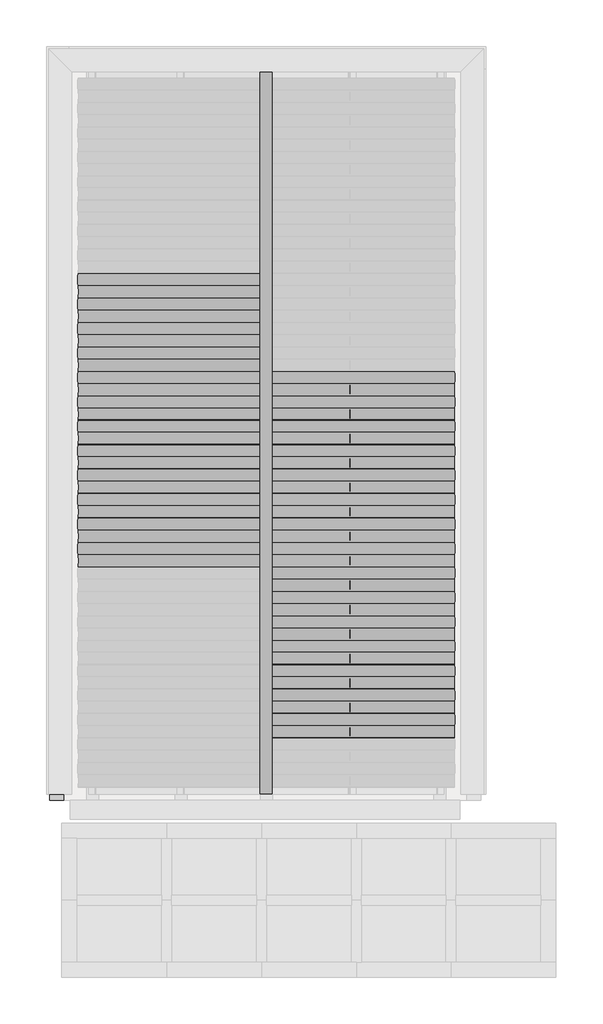
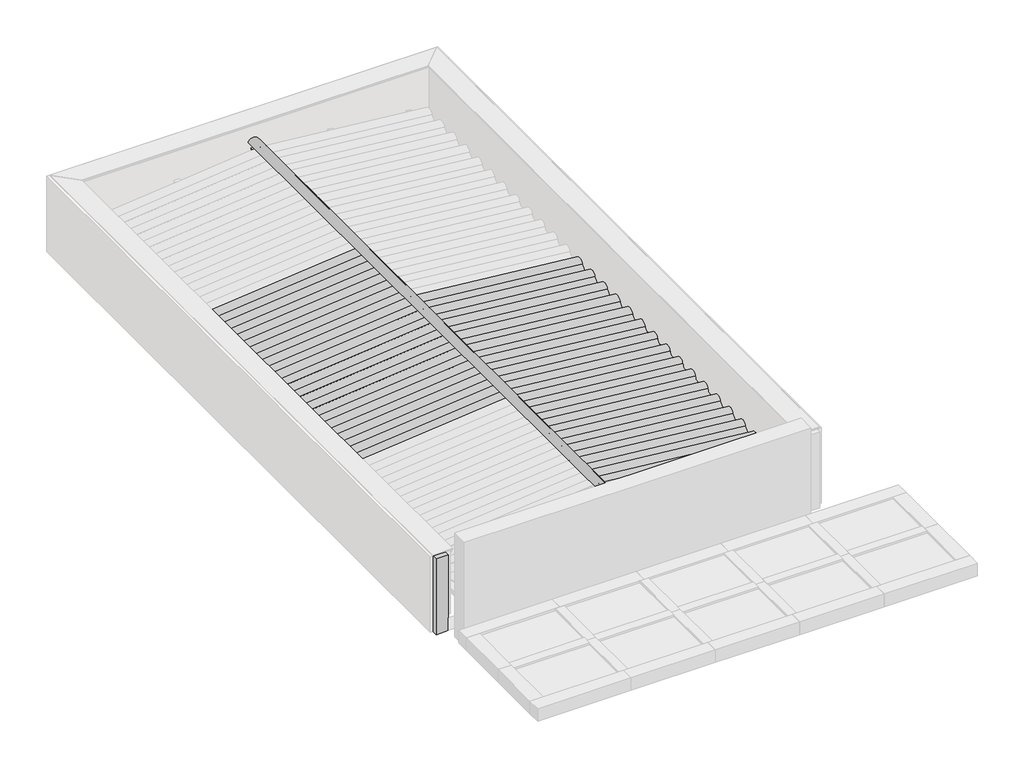
# One storey, part 2 of 3: 35 beams, 6 columns.
"""IFC4 building model written with IfcOpenShell, lengths in millimetres."""

import ifcopenshell
import ifcopenshell.guid

model = None  # the IFC model being written
_history = None  # IfcOwnerHistory: only IFC2X3 demands one
_inside = {}  # id of a spatial element -> (the spatial element, [elements in it])
_under = {}  # id of a project, library or spatial element -> (it, [spatial elements below it])
_declared = {}  # id of a project -> (the project, [libraries it declares])
_typed = {}  # id of a type object -> (the type object, [elements of that type])
_made_of = {}  # id of a material, layer set ... -> (it, [elements and type objects made of it])


def new_model(schema):
    """Start an empty IFC model of exactly this schema.

    Asked for "IFC4X3", IfcOpenShell would pick the latest addendum, in which some entities
    have other attributes; the version numbers below select the first issue.
    IFC2X3 requires an IfcOwnerHistory on every rooted entity: one is made here for all.
    """
    global model, _history
    if schema == "IFC4X3":
        model = ifcopenshell.file(schema_version=(4, 3, 0, 0))
    else:
        model = ifcopenshell.file(schema=schema)
    _inside.clear()
    _under.clear()
    _declared.clear()
    _typed.clear()
    _made_of.clear()
    _history = None
    if model.schema == "IFC2X3":
        org = make("IfcOrganization", Name="unknown")
        user = make(
            "IfcPersonAndOrganization",
            ThePerson=make("IfcPerson", FamilyName="unknown"),
            TheOrganization=org,
        )
        app = make(
            "IfcApplication",
            ApplicationDeveloper=org,
            Version="unknown",
            ApplicationFullName="unknown",
            ApplicationIdentifier="unknown",
        )
        _history = make(
            "IfcOwnerHistory",
            OwningUser=user,
            OwningApplication=app,
            ChangeAction="ADDED",
            CreationDate=0,
        )
    return model


def make(cls, **values):
    """One entity of the class cls with the attributes given. An attribute that is None is left unset."""
    return model.create_entity(
        cls, **{name: value for name, value in values.items() if value is not None}
    )


def rooted(cls, **values):
    """An entity with a GlobalId (a new one), such as an element, a storey or a relation."""
    return make(cls, GlobalId=ifcopenshell.guid.new(), OwnerHistory=_history, **values)


def si_unit(unit_type, name, prefix=None):
    """IfcSIUnit, for example si_unit("LENGTHUNIT", "METRE", prefix="MILLI")."""
    return make("IfcSIUnit", UnitType=unit_type, Prefix=prefix, Name=name)


def assignment(units):
    """IfcUnitAssignment: the units of a project."""
    return None if units is None else make("IfcUnitAssignment", Units=units)


def point(xyz):
    """IfcCartesianPoint."""
    return None if xyz is None else make("IfcCartesianPoint", Coordinates=xyz)


def direction(xyz):
    """IfcDirection."""
    return None if xyz is None else make("IfcDirection", DirectionRatios=xyz)


def frame(location, z_axis=None, x_axis=None):
    """IfcAxis2Placement3D, a coordinate frame: its origin and axes. An axis left out is left unset."""
    return make(
        "IfcAxis2Placement3D",
        Location=point(location),
        Axis=direction(z_axis),
        RefDirection=direction(x_axis),
    )


def frame_2d(location, x_axis=None):
    """IfcAxis2Placement2D, a coordinate frame in the plane: its origin and x axis."""
    return make(
        "IfcAxis2Placement2D", Location=point(location), RefDirection=direction(x_axis)
    )


def origin():
    """The frame at (0, 0, 0) with its axes left unset."""
    return frame((0.0, 0.0, 0.0))


def place(relative_to, where):
    """IfcLocalPlacement: puts the frame where relative to a parent placement (None: the world)."""
    return make(
        "IfcLocalPlacement", PlacementRelTo=relative_to, RelativePlacement=where
    )


def context(
    kind, dimensions, precision=None, world=None, true_north=None, identifier=None
):
    """IfcGeometricRepresentationContext, for example the 3D "Model" context."""
    return make(
        "IfcGeometricRepresentationContext",
        ContextIdentifier=identifier,
        ContextType=kind,
        CoordinateSpaceDimension=dimensions,
        Precision=precision,
        WorldCoordinateSystem=world,
        TrueNorth=true_north,
    )


def project(units=None, contexts=None):
    """IfcProject with its units and contexts."""
    return rooted(
        "IfcProject",
        Name="project",
        RepresentationContexts=contexts,
        UnitsInContext=assignment(units),
    )


def spatial(cls, under=None, at=None, **own):
    """A site, building, storey or space (cls), placed at a placement, below another one or the project."""
    s = rooted(cls, ObjectPlacement=at, **own)
    if under is not None:
        _under.setdefault(under.id(), (under, []))[1].append(s)
    return s


def polyline(points):
    """IfcPolyline through the points."""
    return make("IfcPolyline", Points=[point(p) for p in points])


def circle_curve(where, radius):
    """IfcCircle in the frame where."""
    return make("IfcCircle", Position=where, Radius=radius)


def trimmed(basis, trim1, trim2, sense, master):
    """IfcTrimmedCurve: the piece of a basis curve between two trims."""
    return make(
        "IfcTrimmedCurve",
        BasisCurve=basis,
        Trim1=trim1,
        Trim2=trim2,
        SenseAgreement=sense,
        MasterRepresentation=master,
    )


def segment(curve, same_sense, transition):
    """IfcCompositeCurveSegment."""
    return make(
        "IfcCompositeCurveSegment",
        Transition=transition,
        SameSense=same_sense,
        ParentCurve=curve,
    )


def composite_curve(segments, self_intersect=None):
    """IfcCompositeCurve: segments joined end to end."""
    return make("IfcCompositeCurve", Segments=segments, SelfIntersect=self_intersect)


def outline(outer, holes=None, kind="AREA"):
    """IfcArbitraryClosedProfileDef: a profile drawn as a closed curve; with holes, ...WithVoids."""
    if holes is None:
        return make("IfcArbitraryClosedProfileDef", ProfileType=kind, OuterCurve=outer)
    return make(
        "IfcArbitraryProfileDefWithVoids",
        ProfileType=kind,
        OuterCurve=outer,
        InnerCurves=holes,
    )


def extrude(swept, where, along, depth):
    """IfcExtrudedAreaSolid: the profile swept, set in the frame where, extruded along a direction by depth."""
    return make(
        "IfcExtrudedAreaSolid",
        SweptArea=swept,
        Position=where,
        ExtrudedDirection=direction(along),
        Depth=depth,
    )


def faces_of(points, faces, orient=None, outer=None):
    """IfcFace entities. A face is a list of loops; a loop is a list of indices into points, from 0.

    orient and outer hold one flag for each loop. By default every Orientation is true, the
    first loop of a face is its IfcFaceOuterBound and the others are IfcFaceBound.
    """
    made = []
    for i, loops in enumerate(faces):
        bounds = []
        for j, loop in enumerate(loops):
            is_outer = j == 0 if outer is None else outer[i][j]
            bounds.append(
                make(
                    "IfcFaceOuterBound" if is_outer else "IfcFaceBound",
                    Bound=make("IfcPolyLoop", Polygon=[points[k] for k in loop]),
                    Orientation=True if orient is None else orient[i][j],
                )
            )
        made.append(make("IfcFace", Bounds=bounds))
    return made


def faceted_brep(points, faces, orient=None, outer=None, voids=None):
    """IfcFacetedBrep: a solid bounded by flat faces; with voids (closed shells), ...WithVoids."""
    shared = [point(p) for p in points]
    hull = make("IfcClosedShell", CfsFaces=faces_of(shared, faces, orient, outer))
    if voids is None:
        return make("IfcFacetedBrep", Outer=hull)
    return make(
        "IfcFacetedBrepWithVoids",
        Outer=hull,
        Voids=[
            make(cls, CfsFaces=faces_of(shared, fs, o, b)) for cls, fs, o, b in voids
        ],
    )


def shape(context_of_items, identifier, shape_type, items):
    """IfcShapeRepresentation: the items that make up one representation, for example the "Body"."""
    return make(
        "IfcShapeRepresentation",
        ContextOfItems=context_of_items,
        RepresentationIdentifier=identifier,
        RepresentationType=shape_type,
        Items=items,
    )


def source(mapping_origin, context_of_items, identifier, shape_type, items):
    """IfcRepresentationMap: a shape defined once, which mapped items show again and again."""
    return make(
        "IfcRepresentationMap",
        MappingOrigin=mapping_origin,
        MappedRepresentation=shape(context_of_items, identifier, shape_type, items),
    )


def transform(
    local_origin,
    x_axis=None,
    y_axis=None,
    z_axis=None,
    scale=None,
    scale2=None,
    scale3=None,
    uniform=True,
):
    """IfcCartesianTransformationOperator3D, or its non-uniform kind. x_axis, y_axis, z_axis: its Axis1, 2, 3."""
    if uniform:
        return make(
            "IfcCartesianTransformationOperator3D",
            Axis1=direction(x_axis),
            Axis2=direction(y_axis),
            LocalOrigin=point(local_origin),
            Scale=scale,
            Axis3=direction(z_axis),
        )
    return make(
        "IfcCartesianTransformationOperator3DnonUniform",
        Axis1=direction(x_axis),
        Axis2=direction(y_axis),
        LocalOrigin=point(local_origin),
        Scale=scale,
        Axis3=direction(z_axis),
        Scale2=scale2,
        Scale3=scale3,
    )


def mapped(mapping_source, mapping_target):
    """IfcMappedItem: shows the shape of a source again, moved by a transform."""
    return make(
        "IfcMappedItem", MappingSource=mapping_source, MappingTarget=mapping_target
    )


def made_of(thing, what):
    """Note that an element or type object is made of a material, layer set ...; save() writes the relation."""
    if what is not None:
        _made_of.setdefault(what.id(), (what, []))[1].append(thing)
    return thing


def element(
    cls,
    number,
    at=None,
    inside=None,
    cuts=None,
    type_object=None,
    material=None,
    context=None,
    identifier="Body",
    shape_type=None,
    held_by="IfcProductDefinitionShape",
    body=None,
    shapes=None,
    **own,
):
    """One element of the class cls, such as IfcWall. Its Tag is "e" and its number.

    at: its placement. inside: the storey or other place that contains it. cuts: it is an
    opening in that element (IfcRelVoidsElement). A single representation is given by context,
    identifier, shape_type and body (its items); several are given by shapes. held_by: the class
    of the entity that holds the representations. save() writes the other relations.
    """
    e = rooted(cls, Tag="e%d" % number, ObjectPlacement=at, **own)
    if body is not None:
        shapes = [shape(context, identifier, shape_type, body)]
    if shapes is not None:
        e.Representation = make(held_by, Representations=shapes)
    if inside is not None:
        _inside.setdefault(inside.id(), (inside, []))[1].append(e)
    if cuts is not None:
        rooted(
            "IfcRelVoidsElement", RelatingBuildingElement=cuts, RelatedOpeningElement=e
        )
    if type_object is not None:
        _typed.setdefault(type_object.id(), (type_object, []))[1].append(e)
    return made_of(e, material)


def aggregate(whole, parts):
    """IfcRelAggregates: a whole, such as a stair, and the parts it consists of."""
    return rooted("IfcRelAggregates", RelatingObject=whole, RelatedObjects=parts)


def save(model, path):
    """Write the relations noted so far, then the file.

    IfcRelAggregates (storeys below a building ...), IfcRelContainedInSpatialStructure (elements
    in a storey), IfcRelDefinesByType, IfcRelAssociatesMaterial and IfcRelDeclares: one each for
    every whole, place, type object, material and project.
    """
    for whole, parts in _under.values():
        aggregate(whole, parts)
    for where, things in _inside.values():
        rooted(
            "IfcRelContainedInSpatialStructure",
            RelatedElements=things,
            RelatingStructure=where,
        )
    for kind, things in _typed.values():
        rooted("IfcRelDefinesByType", RelatedObjects=things, RelatingType=kind)
    for what, things in _made_of.values():
        rooted("IfcRelAssociatesMaterial", RelatedObjects=things, RelatingMaterial=what)
    for by, libraries in _declared.values():
        rooted("IfcRelDeclares", RelatingContext=by, RelatedDefinitions=libraries)
    model.write(path)


def cumeeira_telha_ondulada_fibrocimento_28917381(model_context):
    return source(origin(), model_context, "Body", "SweptSolid", [
        extrude(outline(composite_curve([segment(polyline([(58.3970135, 42.4437972), (53.9055884, 40.2467307)]), True, "CONTINUOUS"), segment(trimmed(circle_curve(frame_2d((-1.6029865, 13.0936483)), 61.7939461), [point((53.9055884, 40.2467307))], [point((-57.1115615, 40.2467307))], True, "CARTESIAN"), True, "CONTINUOUS"), segment(polyline([(-57.1115615, 40.2467307), (-61.6029865, 42.4437972)]), True, "CONTINUOUS"), segment(trimmed(circle_curve(frame_2d((-1.6029865, 13.0936483)), 66.7939461), [point((-61.6029865, 42.4437972))], [point((58.3970135, 42.4437972))], False, "CARTESIAN"), True, "CONTINUOUS")], self_intersect=False)), frame((-3626.5, 0.0, 0.0), z_axis=(1.0, 0.0, 0.0), x_axis=(0.0, 1.0, 0.0)), (0.0, 0.0, 1.0), 7253.0),
    ])


def viga_cumeeira_6x16cm_d80f05ee(model_context):
    return source(origin(), model_context, "Body", "SweptSolid", [
        extrude(outline(polyline([(3626.5, 30.0), (3626.5, -30.0), (-3626.5, -30.0), (-3626.5, 30.0), (3626.5, 30.0)])), frame((0.0, 0.0, -80.0), z_axis=(0.0, 0.0, 1.0), x_axis=(1.0, 0.0, 0.0)), (0.0, 0.0, 1.0), 160.0),
    ])


def column_1cffec27(model_context):
    return source(origin(), model_context, "Body", "SweptSolid", [
        extrude(outline(polyline([(30.0, 80.0), (30.0, -80.0), (-30.0, -80.0), (-30.0, 80.0), (30.0, 80.0)])), frame((0.0, 0.0, 3110.0), z_axis=(0.0, 0.0, 1.0), x_axis=(1.0, 0.0, 0.0)), (0.0, 0.0, 1.0), 238.0),
    ])


def column_35730ad5(model_context):
    return source(origin(), model_context, "Body", "SweptSolid", [
        extrude(outline(polyline([(30.0, 80.0), (30.0, -80.0), (-30.0, -80.0), (-30.0, 80.0), (30.0, 80.0)])), frame((0.0, 0.0, 3110.0), z_axis=(0.0, 0.0, 1.0), x_axis=(1.0, 0.0, 0.0)), (0.0, 0.0, 1.0), 197.9),
    ])


def column_00c463e4(model_context):
    return source(origin(), model_context, "Body", "SweptSolid", [
        extrude(outline(polyline([(30.0, 80.0), (30.0, -80.0), (-30.0, -80.0), (-30.0, 80.0), (30.0, 80.0)])), frame((0.0, 0.0, 3110.0), z_axis=(0.0, 0.0, 1.0), x_axis=(1.0, 0.0, 0.0)), (0.0, 0.0, 1.0), 109.8),
    ])


model = new_model("IFC4")

# Units and contexts
model_context = context("Model", 3, world=origin())
ifc_project = project(units=[si_unit("LENGTHUNIT", "METRE", prefix="MILLI")], contexts=[model_context])

# Site, building, storey
site = spatial("IfcSite", under=ifc_project)
building = spatial("IfcBuilding", under=site)
storey = spatial("IfcBuildingStorey", under=building, Name="COB. GARAGEM", Elevation=3050.0)

# Beams
placement = place(None, origin())
element("IfcBeam", 1, ObjectType="Madeira de lei : Berço 6x12cm", at=placement, inside=storey, context=model_context, shape_type="SweptSolid", body=[
    extrude(outline(polyline([(-9620.281307, 4423.9300153), (-9500.281307, 4423.9300153), (-9500.281307, 2423.9300153), (-9620.281307, 2423.9300153), (-9620.281307, 4423.9300153)])), frame((0.0, 0.0, 3050.0), z_axis=(0.0, 0.0, 1.0), x_axis=(1.0, 0.0, 0.0)), (0.0, 0.0, 1.0), 60.0),
])
element("IfcBeam", 2, ObjectType="Madeira de lei : Berço 6x12cm", at=placement, inside=storey, context=model_context, shape_type="SweptSolid", body=[
    extrude(outline(polyline([(-9620.281307, 2423.9300153), (-9500.281307, 2423.9300153), (-9500.281307, 423.9300153), (-9620.281307, 423.9300153), (-9620.281307, 2423.9300153)])), frame((0.0, 0.0, 3050.0), z_axis=(0.0, 0.0, 1.0), x_axis=(1.0, 0.0, 0.0)), (0.0, 0.0, 1.0), 60.0),
])
element("IfcBeam", 3, ObjectType="Madeira de lei : Berço 6x12cm", at=placement, inside=storey, context=model_context, shape_type="SweptSolid", body=[
    extrude(outline(polyline([(-8767.0824227, 4423.9300153), (-8647.0824227, 4423.9300153), (-8647.0824227, 2423.9300153), (-8767.0824227, 2423.9300153), (-8767.0824227, 4423.9300153)])), frame((0.0, 0.0, 3050.0), z_axis=(0.0, 0.0, 1.0), x_axis=(1.0, 0.0, 0.0)), (0.0, 0.0, 1.0), 60.0),
])
element("IfcBeam", 4, ObjectType="Madeira de lei : Berço 6x12cm", at=placement, inside=storey, context=model_context, shape_type="SweptSolid", body=[
    extrude(outline(polyline([(-10473.4801913, 4423.9300153), (-10353.4801913, 4423.9300153), (-10353.4801913, 2423.9300153), (-10473.4801913, 2423.9300153), (-10473.4801913, 4423.9300153)])), frame((0.0, 0.0, 3050.0), z_axis=(0.0, 0.0, 1.0), x_axis=(1.0, 0.0, 0.0)), (0.0, 0.0, 1.0), 60.0),
])
element("IfcBeam", 5, ObjectType="Madeira de lei : Berço 6x12cm", at=placement, inside=storey, context=model_context, shape_type="SweptSolid", body=[
    extrude(outline(polyline([(-11356.5301913, 4423.9300153), (-11236.5301913, 4423.9300153), (-11236.5301913, 2423.9300153), (-11356.5301913, 2423.9300153), (-11356.5301913, 4423.9300153)])), frame((0.0, 0.0, 3050.0), z_axis=(0.0, 0.0, 1.0), x_axis=(1.0, 0.0, 0.0)), (0.0, 0.0, 1.0), 60.0),
])
cumeeira_telha_ondulada_fibrocimento_shape = cumeeira_telha_ondulada_fibrocimento_28917381(model_context)
element("IfcBeam", 6, ObjectType="Cumeeira Telha Ondulada : Fibrocimento", at=placement, inside=storey, context=model_context, shape_type="MappedRepresentation", body=[
    mapped(cumeeira_telha_ondulada_fibrocimento_shape, transform((-9560.281307, 3455.9300153, 3545.9751229), x_axis=(0.0, -1.0, 0.0), y_axis=(1.0, 0.0, 0.0), z_axis=(0.0, 0.0, 1.0))),
])
element("IfcBeam", 7, ObjectType="TQS - Viga retangular : 14.0 x 90.0", at=placement, inside=storey, context=model_context, shape_type="Brep", body=[
    faceted_brep([(-11590.281307, 7084.4300153, 3800.0), (-11730.281307, 7084.4300153, 3800.0), (-11730.281307, -234.5699847, 3800.0), (-11590.281307, -234.5699847, 3800.0), (-11590.281307, 7084.4300153, 2900.0), (-11590.281307, 7084.4300153, 3050.0), (-11590.281307, -234.5699847, 3050.0), (-11590.281307, -234.5699847, 2900.0), (-11730.281307, 7084.4300153, 2900.0), (-11730.281307, -234.5699847, 2900.0)], [[[0, 1, 2, 3]], [[4, 5, 0, 3, 6, 7]], [[8, 4, 7, 9]], [[1, 8, 9, 2]], [[2, 9, 7, 6, 3]], [[1, 0, 5, 4, 8]]]),
])
element("IfcBeam", 8, ObjectType="Telha Ondulada : Fibrocimento", at=placement, inside=storey, context=model_context, shape_type="SweptSolid", body=[
    extrude(outline(composite_curve([segment(trimmed(circle_curve(frame_2d((-58.7002979, -53.2060538)), 66.7939461), [point((-29.350149, 6.7939462))], [point((-29.350149, -113.2060538))], False, "CARTESIAN"), True, "CONTINUOUS"), segment(polyline([(-29.350149, -113.2060538), (-31.5472155, -108.7146288)]), True, "CONTINUOUS"), segment(trimmed(circle_curve(frame_2d((-58.7002979, -53.2060538)), 61.7939461), [point((-31.5472155, -108.7146288))], [point((-31.5472155, 2.3025211))], True, "CARTESIAN"), True, "CONTINUOUS"), segment(trimmed(circle_curve(frame_2d((0.0, 66.7939462)), 71.7939461), [point((-31.5472155, 2.3025211))], [point((-31.5472155, 131.2853712))], False, "CARTESIAN"), True, "CONTINUOUS"), segment(polyline([(-31.5472155, 131.2853712), (-29.350149, 126.7939462)]), True, "CONTINUOUS"), segment(trimmed(circle_curve(frame_2d((0.0, 66.7939462)), 66.7939461), [point((-29.350149, 126.7939462))], [point((-29.350149, 6.7939462))], True, "CARTESIAN"), True, "CONTINUOUS")], self_intersect=False)), frame((-11446.918865, 2229.326948, 3394.3067746), z_axis=(0.9950371902099892, 0.0, 0.09950371902099919), x_axis=(-0.09950371902099919, 0.0, 0.9950371902099892)), (0.0, 0.0, 1.0), 1886.8678854),
])
element("IfcBeam", 9, ObjectType="Telha Ondulada : Fibrocimento", at=placement, inside=storey, context=model_context, shape_type="SweptSolid", body=[
    extrude(outline(composite_curve([segment(trimmed(circle_curve(frame_2d((-58.7002979, -53.2060538)), 66.7939461), [point((-29.350149, 6.7939462))], [point((-29.350149, -113.2060538))], False, "CARTESIAN"), True, "CONTINUOUS"), segment(polyline([(-29.350149, -113.2060538), (-31.5472155, -108.7146288)]), True, "CONTINUOUS"), segment(trimmed(circle_curve(frame_2d((-58.7002979, -53.2060538)), 61.7939461), [point((-31.5472155, -108.7146288))], [point((-31.5472155, 2.3025211))], True, "CARTESIAN"), True, "CONTINUOUS"), segment(trimmed(circle_curve(frame_2d((0.0, 66.7939462)), 71.7939461), [point((-31.5472155, 2.3025211))], [point((-31.5472155, 131.2853712))], False, "CARTESIAN"), True, "CONTINUOUS"), segment(polyline([(-31.5472155, 131.2853712), (-29.350149, 126.7939462)]), True, "CONTINUOUS"), segment(trimmed(circle_curve(frame_2d((0.0, 66.7939462)), 66.7939461), [point((-29.350149, 126.7939462))], [point((-29.350149, 6.7939462))], True, "CARTESIAN"), True, "CONTINUOUS")], self_intersect=False)), frame((-11446.918865, 2473.826948, 3394.3067746), z_axis=(0.9950371902099892, 0.0, 0.09950371902099932), x_axis=(-0.09950371902099932, 0.0, 0.9950371902099892)), (0.0, 0.0, 1.0), 1886.8678854),
])
element("IfcBeam", 10, ObjectType="Telha Ondulada : Fibrocimento", at=placement, inside=storey, context=model_context, shape_type="SweptSolid", body=[
    extrude(outline(composite_curve([segment(trimmed(circle_curve(frame_2d((-58.7002979, -53.2060538)), 66.7939461), [point((-29.350149, 6.7939462))], [point((-29.350149, -113.2060538))], False, "CARTESIAN"), True, "CONTINUOUS"), segment(polyline([(-29.350149, -113.2060538), (-31.5472155, -108.7146288)]), True, "CONTINUOUS"), segment(trimmed(circle_curve(frame_2d((-58.7002979, -53.2060538)), 61.7939461), [point((-31.5472155, -108.7146288))], [point((-31.5472155, 2.3025211))], True, "CARTESIAN"), True, "CONTINUOUS"), segment(trimmed(circle_curve(frame_2d((0.0, 66.7939462)), 71.7939461), [point((-31.5472155, 2.3025211))], [point((-31.5472155, 131.2853712))], False, "CARTESIAN"), True, "CONTINUOUS"), segment(polyline([(-31.5472155, 131.2853712), (-29.350149, 126.7939462)]), True, "CONTINUOUS"), segment(trimmed(circle_curve(frame_2d((0.0, 66.7939462)), 66.7939461), [point((-29.350149, 126.7939462))], [point((-29.350149, 6.7939462))], True, "CARTESIAN"), True, "CONTINUOUS")], self_intersect=False)), frame((-11446.918865, 2718.326948, 3394.3067746), z_axis=(0.9950371902099892, 0.0, 0.09950371902099937), x_axis=(-0.09950371902099937, 0.0, 0.9950371902099892)), (0.0, 0.0, 1.0), 1886.8678854),
])
element("IfcBeam", 11, ObjectType="Telha Ondulada : Fibrocimento", at=placement, inside=storey, context=model_context, shape_type="SweptSolid", body=[
    extrude(outline(composite_curve([segment(trimmed(circle_curve(frame_2d((-58.7002979, -53.2060538)), 66.7939461), [point((-29.350149, 6.7939462))], [point((-29.350149, -113.2060538))], False, "CARTESIAN"), True, "CONTINUOUS"), segment(polyline([(-29.350149, -113.2060538), (-31.5472155, -108.7146288)]), True, "CONTINUOUS"), segment(trimmed(circle_curve(frame_2d((-58.7002979, -53.2060538)), 61.7939461), [point((-31.5472155, -108.7146288))], [point((-31.5472155, 2.3025211))], True, "CARTESIAN"), True, "CONTINUOUS"), segment(trimmed(circle_curve(frame_2d((0.0, 66.7939462)), 71.7939461), [point((-31.5472155, 2.3025211))], [point((-31.5472155, 131.2853712))], False, "CARTESIAN"), True, "CONTINUOUS"), segment(polyline([(-31.5472155, 131.2853712), (-29.350149, 126.7939462)]), True, "CONTINUOUS"), segment(trimmed(circle_curve(frame_2d((0.0, 66.7939462)), 66.7939461), [point((-29.350149, 126.7939462))], [point((-29.350149, 6.7939462))], True, "CARTESIAN"), True, "CONTINUOUS")], self_intersect=False)), frame((-11446.918865, 2962.826948, 3394.3067746), z_axis=(0.9950371902099892, 0.0, 0.09950371902099943), x_axis=(-0.09950371902099943, 0.0, 0.9950371902099892)), (0.0, 0.0, 1.0), 1886.8678854),
])
element("IfcBeam", 12, ObjectType="Telha Ondulada : Fibrocimento", at=placement, inside=storey, context=model_context, shape_type="SweptSolid", body=[
    extrude(outline(composite_curve([segment(trimmed(circle_curve(frame_2d((-58.7002979, -53.2060538)), 66.7939461), [point((-29.350149, 6.7939462))], [point((-29.350149, -113.2060538))], False, "CARTESIAN"), True, "CONTINUOUS"), segment(polyline([(-29.350149, -113.2060538), (-31.5472155, -108.7146288)]), True, "CONTINUOUS"), segment(trimmed(circle_curve(frame_2d((-58.7002979, -53.2060538)), 61.7939461), [point((-31.5472155, -108.7146288))], [point((-31.5472155, 2.3025211))], True, "CARTESIAN"), True, "CONTINUOUS"), segment(trimmed(circle_curve(frame_2d((0.0, 66.7939462)), 71.7939461), [point((-31.5472155, 2.3025211))], [point((-31.5472155, 131.2853712))], False, "CARTESIAN"), True, "CONTINUOUS"), segment(polyline([(-31.5472155, 131.2853712), (-29.350149, 126.7939462)]), True, "CONTINUOUS"), segment(trimmed(circle_curve(frame_2d((0.0, 66.7939462)), 66.7939461), [point((-29.350149, 126.7939462))], [point((-29.350149, 6.7939462))], True, "CARTESIAN"), True, "CONTINUOUS")], self_intersect=False)), frame((-11446.918865, 3207.326948, 3394.3067746), z_axis=(0.9950371902099892, 0.0, 0.09950371902099954), x_axis=(-0.09950371902099954, 0.0, 0.9950371902099892)), (0.0, 0.0, 1.0), 1886.8678854),
])
element("IfcBeam", 13, ObjectType="Telha Ondulada : Fibrocimento", at=placement, inside=storey, context=model_context, shape_type="SweptSolid", body=[
    extrude(outline(composite_curve([segment(trimmed(circle_curve(frame_2d((-58.7002979, -53.2060538)), 66.7939461), [point((-29.350149, 6.7939462))], [point((-29.350149, -113.2060538))], False, "CARTESIAN"), True, "CONTINUOUS"), segment(polyline([(-29.350149, -113.2060538), (-31.5472155, -108.7146288)]), True, "CONTINUOUS"), segment(trimmed(circle_curve(frame_2d((-58.7002979, -53.2060538)), 61.7939461), [point((-31.5472155, -108.7146288))], [point((-31.5472155, 2.3025211))], True, "CARTESIAN"), True, "CONTINUOUS"), segment(trimmed(circle_curve(frame_2d((0.0, 66.7939462)), 71.7939461), [point((-31.5472155, 2.3025211))], [point((-31.5472155, 131.2853712))], False, "CARTESIAN"), True, "CONTINUOUS"), segment(polyline([(-31.5472155, 131.2853712), (-29.350149, 126.7939462)]), True, "CONTINUOUS"), segment(trimmed(circle_curve(frame_2d((0.0, 66.7939462)), 66.7939461), [point((-29.350149, 126.7939462))], [point((-29.350149, 6.7939462))], True, "CARTESIAN"), True, "CONTINUOUS")], self_intersect=False)), frame((-11446.918865, 3451.826948, 3394.3067746), z_axis=(0.9950371902099892, 0.0, 0.09950371902099937), x_axis=(-0.09950371902099937, 0.0, 0.9950371902099892)), (0.0, 0.0, 1.0), 1886.8678854),
])
element("IfcBeam", 14, ObjectType="Telha Ondulada : Fibrocimento", at=placement, inside=storey, context=model_context, shape_type="SweptSolid", body=[
    extrude(outline(composite_curve([segment(trimmed(circle_curve(frame_2d((-58.7002979, -53.2060538)), 66.7939461), [point((-29.350149, 6.7939462))], [point((-29.350149, -113.2060538))], False, "CARTESIAN"), True, "CONTINUOUS"), segment(polyline([(-29.350149, -113.2060538), (-31.5472155, -108.7146288)]), True, "CONTINUOUS"), segment(trimmed(circle_curve(frame_2d((-58.7002979, -53.2060538)), 61.7939461), [point((-31.5472155, -108.7146288))], [point((-31.5472155, 2.3025211))], True, "CARTESIAN"), True, "CONTINUOUS"), segment(trimmed(circle_curve(frame_2d((0.0, 66.7939462)), 71.7939461), [point((-31.5472155, 2.3025211))], [point((-31.5472155, 131.2853712))], False, "CARTESIAN"), True, "CONTINUOUS"), segment(polyline([(-31.5472155, 131.2853712), (-29.350149, 126.7939462)]), True, "CONTINUOUS"), segment(trimmed(circle_curve(frame_2d((0.0, 66.7939462)), 66.7939461), [point((-29.350149, 126.7939462))], [point((-29.350149, 6.7939462))], True, "CARTESIAN"), True, "CONTINUOUS")], self_intersect=False)), frame((-11446.918865, 3696.326948, 3394.3067746), z_axis=(0.9950371902099892, 0.0, 0.09950371902099914), x_axis=(-0.09950371902099914, 0.0, 0.9950371902099892)), (0.0, 0.0, 1.0), 1886.8678854),
])
element("IfcBeam", 15, ObjectType="Telha Ondulada : Fibrocimento", at=placement, inside=storey, context=model_context, shape_type="SweptSolid", body=[
    extrude(outline(composite_curve([segment(trimmed(circle_curve(frame_2d((-58.7002979, -53.2060538)), 66.7939461), [point((-29.350149, 6.7939462))], [point((-29.350149, -113.2060538))], False, "CARTESIAN"), True, "CONTINUOUS"), segment(polyline([(-29.350149, -113.2060538), (-31.5472155, -108.7146288)]), True, "CONTINUOUS"), segment(trimmed(circle_curve(frame_2d((-58.7002979, -53.2060538)), 61.7939461), [point((-31.5472155, -108.7146288))], [point((-31.5472155, 2.3025211))], True, "CARTESIAN"), True, "CONTINUOUS"), segment(trimmed(circle_curve(frame_2d((0.0, 66.7939462)), 71.7939461), [point((-31.5472155, 2.3025211))], [point((-31.5472155, 131.2853712))], False, "CARTESIAN"), True, "CONTINUOUS"), segment(polyline([(-31.5472155, 131.2853712), (-29.350149, 126.7939462)]), True, "CONTINUOUS"), segment(trimmed(circle_curve(frame_2d((0.0, 66.7939462)), 66.7939461), [point((-29.350149, 126.7939462))], [point((-29.350149, 6.7939462))], True, "CARTESIAN"), True, "CONTINUOUS")], self_intersect=False)), frame((-11446.918865, 3940.826948, 3394.3067746), z_axis=(0.9950371902099892, 0.0, 0.09950371902099948), x_axis=(-0.09950371902099948, 0.0, 0.9950371902099892)), (0.0, 0.0, 1.0), 1886.8678854),
])
element("IfcBeam", 16, ObjectType="Telha Ondulada : Fibrocimento", at=placement, inside=storey, context=model_context, shape_type="SweptSolid", body=[
    extrude(outline(composite_curve([segment(trimmed(circle_curve(frame_2d((-58.7002979, -53.2060538)), 66.7939461), [point((-29.350149, 6.7939462))], [point((-29.350149, -113.2060538))], False, "CARTESIAN"), True, "CONTINUOUS"), segment(polyline([(-29.350149, -113.2060538), (-31.5472155, -108.7146288)]), True, "CONTINUOUS"), segment(trimmed(circle_curve(frame_2d((-58.7002979, -53.2060538)), 61.7939461), [point((-31.5472155, -108.7146288))], [point((-31.5472155, 2.3025211))], True, "CARTESIAN"), True, "CONTINUOUS"), segment(trimmed(circle_curve(frame_2d((0.0, 66.7939462)), 71.7939461), [point((-31.5472155, 2.3025211))], [point((-31.5472155, 131.2853712))], False, "CARTESIAN"), True, "CONTINUOUS"), segment(polyline([(-31.5472155, 131.2853712), (-29.350149, 126.7939462)]), True, "CONTINUOUS"), segment(trimmed(circle_curve(frame_2d((0.0, 66.7939462)), 66.7939461), [point((-29.350149, 126.7939462))], [point((-29.350149, 6.7939462))], True, "CARTESIAN"), True, "CONTINUOUS")], self_intersect=False)), frame((-11446.918865, 4185.326948, 3394.3067746), z_axis=(0.9950371902099892, 0.0, 0.09950371902099932), x_axis=(-0.09950371902099932, 0.0, 0.9950371902099892)), (0.0, 0.0, 1.0), 1886.8678854),
])
element("IfcBeam", 17, ObjectType="Telha Ondulada : Fibrocimento", at=placement, inside=storey, context=model_context, shape_type="SweptSolid", body=[
    extrude(outline(composite_curve([segment(trimmed(circle_curve(frame_2d((-58.7002979, -53.2060538)), 66.7939461), [point((-29.350149, 6.7939462))], [point((-29.350149, -113.2060538))], False, "CARTESIAN"), True, "CONTINUOUS"), segment(polyline([(-29.350149, -113.2060538), (-31.5472155, -108.7146288)]), True, "CONTINUOUS"), segment(trimmed(circle_curve(frame_2d((-58.7002979, -53.2060538)), 61.7939461), [point((-31.5472155, -108.7146288))], [point((-31.5472155, 2.3025211))], True, "CARTESIAN"), True, "CONTINUOUS"), segment(trimmed(circle_curve(frame_2d((0.0, 66.7939462)), 71.7939461), [point((-31.5472155, 2.3025211))], [point((-31.5472155, 131.2853712))], False, "CARTESIAN"), True, "CONTINUOUS"), segment(polyline([(-31.5472155, 131.2853712), (-29.350149, 126.7939462)]), True, "CONTINUOUS"), segment(trimmed(circle_curve(frame_2d((0.0, 66.7939462)), 66.7939461), [point((-29.350149, 126.7939462))], [point((-29.350149, 6.7939462))], True, "CARTESIAN"), True, "CONTINUOUS")], self_intersect=False)), frame((-11446.918865, 4429.826948, 3394.3067746), z_axis=(0.9950371902099892, 0.0, 0.09950371902099943), x_axis=(-0.09950371902099943, 0.0, 0.9950371902099892)), (0.0, 0.0, 1.0), 1886.8678854),
])
element("IfcBeam", 18, ObjectType="Telha Ondulada : Fibrocimento", at=placement, inside=storey, context=model_context, shape_type="SweptSolid", body=[
    extrude(outline(composite_curve([segment(trimmed(circle_curve(frame_2d((-58.7002979, -53.2060538)), 66.7939461), [point((-29.350149, 6.7939462))], [point((-29.350149, -113.2060538))], False, "CARTESIAN"), True, "CONTINUOUS"), segment(polyline([(-29.350149, -113.2060538), (-31.5472155, -108.7146288)]), True, "CONTINUOUS"), segment(trimmed(circle_curve(frame_2d((-58.7002979, -53.2060538)), 61.7939461), [point((-31.5472155, -108.7146288))], [point((-31.5472155, 2.3025211))], True, "CARTESIAN"), True, "CONTINUOUS"), segment(trimmed(circle_curve(frame_2d((0.0, 66.7939462)), 71.7939461), [point((-31.5472155, 2.3025211))], [point((-31.5472155, 131.2853712))], False, "CARTESIAN"), True, "CONTINUOUS"), segment(polyline([(-31.5472155, 131.2853712), (-29.350149, 126.7939462)]), True, "CONTINUOUS"), segment(trimmed(circle_curve(frame_2d((0.0, 66.7939462)), 66.7939461), [point((-29.350149, 126.7939462))], [point((-29.350149, 6.7939462))], True, "CARTESIAN"), True, "CONTINUOUS")], self_intersect=False)), frame((-11446.918865, 4674.326948, 3394.3067746), z_axis=(0.9950371902099892, 0.0, 0.09950371902099943), x_axis=(-0.09950371902099943, 0.0, 0.9950371902099892)), (0.0, 0.0, 1.0), 1886.8678854),
])
element("IfcBeam", 19, ObjectType="Telha Ondulada : Fibrocimento", at=placement, inside=storey, context=model_context, shape_type="SweptSolid", body=[
    extrude(outline(composite_curve([segment(trimmed(circle_curve(frame_2d((-58.7002979, -53.2060538)), 66.7939461), [point((-29.350149, 6.7939462))], [point((-29.350149, -113.2060538))], False, "CARTESIAN"), True, "CONTINUOUS"), segment(polyline([(-29.350149, -113.2060538), (-31.5472155, -108.7146288)]), True, "CONTINUOUS"), segment(trimmed(circle_curve(frame_2d((-58.7002979, -53.2060538)), 61.7939461), [point((-31.5472155, -108.7146288))], [point((-31.5472155, 2.3025211))], True, "CARTESIAN"), True, "CONTINUOUS"), segment(trimmed(circle_curve(frame_2d((0.0, 66.7939462)), 71.7939461), [point((-31.5472155, 2.3025211))], [point((-31.5472155, 131.2853712))], False, "CARTESIAN"), True, "CONTINUOUS"), segment(polyline([(-31.5472155, 131.2853712), (-29.350149, 126.7939462)]), True, "CONTINUOUS"), segment(trimmed(circle_curve(frame_2d((0.0, 66.7939462)), 66.7939461), [point((-29.350149, 126.7939462))], [point((-29.350149, 6.7939462))], True, "CARTESIAN"), True, "CONTINUOUS")], self_intersect=False)), frame((-11446.918865, 4918.826948, 3394.3067746), z_axis=(0.9950371902099892, 0.0, 0.09950371902099903), x_axis=(-0.09950371902099903, 0.0, 0.9950371902099892)), (0.0, 0.0, 1.0), 1886.8678854),
])
element("IfcBeam", 20, ObjectType="Telha Ondulada : Fibrocimento", at=placement, inside=storey, context=model_context, shape_type="SweptSolid", body=[
    extrude(outline(composite_curve([segment(trimmed(circle_curve(frame_2d((0.0, 66.7939462)), 66.7939461), [point((29.350149, 6.7939462))], [point((29.350149, 126.7939462))], True, "CARTESIAN"), True, "CONTINUOUS"), segment(polyline([(29.350149, 126.7939462), (31.5472155, 131.2853712)]), True, "CONTINUOUS"), segment(trimmed(circle_curve(frame_2d((0.0, 66.7939462)), 71.7939461), [point((31.5472155, 131.2853712))], [point((31.5472155, 2.3025211))], False, "CARTESIAN"), True, "CONTINUOUS"), segment(trimmed(circle_curve(frame_2d((58.7002979, -53.2060538)), 61.7939461), [point((31.5472155, 2.3025211))], [point((31.5472155, -108.7146288))], True, "CARTESIAN"), True, "CONTINUOUS"), segment(polyline([(31.5472155, -108.7146288), (29.350149, -113.2060538)]), True, "CONTINUOUS"), segment(trimmed(circle_curve(frame_2d((58.7002979, -53.2060538)), 66.7939461), [point((29.350149, -113.2060538))], [point((29.350149, 6.7939462))], False, "CARTESIAN"), True, "CONTINUOUS")], self_intersect=False)), frame((-7673.6437489, 517.826948, 3394.3067746), z_axis=(-0.9950371902099892, 0.0, 0.09950371902099965), x_axis=(-0.09950371902099965, 0.0, -0.9950371902099892)), (0.0, 0.0, 1.0), 1886.8678854),
])
element("IfcBeam", 21, ObjectType="Telha Ondulada : Fibrocimento", at=placement, inside=storey, context=model_context, shape_type="SweptSolid", body=[
    extrude(outline(composite_curve([segment(trimmed(circle_curve(frame_2d((0.0, 66.7939462)), 66.7939461), [point((29.350149, 6.7939462))], [point((29.350149, 126.7939462))], True, "CARTESIAN"), True, "CONTINUOUS"), segment(polyline([(29.350149, 126.7939462), (31.5472155, 131.2853712)]), True, "CONTINUOUS"), segment(trimmed(circle_curve(frame_2d((0.0, 66.7939462)), 71.7939461), [point((31.5472155, 131.2853712))], [point((31.5472155, 2.3025211))], False, "CARTESIAN"), True, "CONTINUOUS"), segment(trimmed(circle_curve(frame_2d((58.7002979, -53.2060538)), 61.7939461), [point((31.5472155, 2.3025211))], [point((31.5472155, -108.7146288))], True, "CARTESIAN"), True, "CONTINUOUS"), segment(polyline([(31.5472155, -108.7146288), (29.350149, -113.2060538)]), True, "CONTINUOUS"), segment(trimmed(circle_curve(frame_2d((58.7002979, -53.2060538)), 66.7939461), [point((29.350149, -113.2060538))], [point((29.350149, 6.7939462))], False, "CARTESIAN"), True, "CONTINUOUS")], self_intersect=False)), frame((-7673.6437489, 762.326948, 3394.3067746), z_axis=(-0.9950371902099892, 0.0, 0.09950371902099965), x_axis=(-0.09950371902099965, 0.0, -0.9950371902099892)), (0.0, 0.0, 1.0), 1886.8678854),
])
element("IfcBeam", 22, ObjectType="Telha Ondulada : Fibrocimento", at=placement, inside=storey, context=model_context, shape_type="SweptSolid", body=[
    extrude(outline(composite_curve([segment(trimmed(circle_curve(frame_2d((0.0, 66.7939462)), 66.7939461), [point((29.350149, 6.7939462))], [point((29.350149, 126.7939462))], True, "CARTESIAN"), True, "CONTINUOUS"), segment(polyline([(29.350149, 126.7939462), (31.5472155, 131.2853712)]), True, "CONTINUOUS"), segment(trimmed(circle_curve(frame_2d((0.0, 66.7939462)), 71.7939461), [point((31.5472155, 131.2853712))], [point((31.5472155, 2.3025211))], False, "CARTESIAN"), True, "CONTINUOUS"), segment(trimmed(circle_curve(frame_2d((58.7002979, -53.2060538)), 61.7939461), [point((31.5472155, 2.3025211))], [point((31.5472155, -108.7146288))], True, "CARTESIAN"), True, "CONTINUOUS"), segment(polyline([(31.5472155, -108.7146288), (29.350149, -113.2060538)]), True, "CONTINUOUS"), segment(trimmed(circle_curve(frame_2d((58.7002979, -53.2060538)), 66.7939461), [point((29.350149, -113.2060538))], [point((29.350149, 6.7939462))], False, "CARTESIAN"), True, "CONTINUOUS")], self_intersect=False)), frame((-7673.6437489, 1006.826948, 3394.3067746), z_axis=(-0.9950371902099892, 0.0, 0.09950371902099965), x_axis=(-0.09950371902099965, 0.0, -0.9950371902099892)), (0.0, 0.0, 1.0), 1886.8678854),
])
element("IfcBeam", 23, ObjectType="Telha Ondulada : Fibrocimento", at=placement, inside=storey, context=model_context, shape_type="SweptSolid", body=[
    extrude(outline(composite_curve([segment(trimmed(circle_curve(frame_2d((0.0, 66.7939462)), 66.7939461), [point((29.350149, 6.7939462))], [point((29.350149, 126.7939462))], True, "CARTESIAN"), True, "CONTINUOUS"), segment(polyline([(29.350149, 126.7939462), (31.5472155, 131.2853712)]), True, "CONTINUOUS"), segment(trimmed(circle_curve(frame_2d((0.0, 66.7939462)), 71.7939461), [point((31.5472155, 131.2853712))], [point((31.5472155, 2.3025211))], False, "CARTESIAN"), True, "CONTINUOUS"), segment(trimmed(circle_curve(frame_2d((58.7002979, -53.2060538)), 61.7939461), [point((31.5472155, 2.3025211))], [point((31.5472155, -108.7146288))], True, "CARTESIAN"), True, "CONTINUOUS"), segment(polyline([(31.5472155, -108.7146288), (29.350149, -113.2060538)]), True, "CONTINUOUS"), segment(trimmed(circle_curve(frame_2d((58.7002979, -53.2060538)), 66.7939461), [point((29.350149, -113.2060538))], [point((29.350149, 6.7939462))], False, "CARTESIAN"), True, "CONTINUOUS")], self_intersect=False)), frame((-7673.6437489, 1251.326948, 3394.3067746), z_axis=(-0.9950371902099892, 0.0, 0.09950371902099965), x_axis=(-0.09950371902099965, 0.0, -0.9950371902099892)), (0.0, 0.0, 1.0), 1886.8678854),
])
element("IfcBeam", 24, ObjectType="Telha Ondulada : Fibrocimento", at=placement, inside=storey, context=model_context, shape_type="SweptSolid", body=[
    extrude(outline(composite_curve([segment(trimmed(circle_curve(frame_2d((0.0, 66.7939462)), 66.7939461), [point((29.350149, 6.7939462))], [point((29.350149, 126.7939462))], True, "CARTESIAN"), True, "CONTINUOUS"), segment(polyline([(29.350149, 126.7939462), (31.5472155, 131.2853712)]), True, "CONTINUOUS"), segment(trimmed(circle_curve(frame_2d((0.0, 66.7939462)), 71.7939461), [point((31.5472155, 131.2853712))], [point((31.5472155, 2.3025211))], False, "CARTESIAN"), True, "CONTINUOUS"), segment(trimmed(circle_curve(frame_2d((58.7002979, -53.2060538)), 61.7939461), [point((31.5472155, 2.3025211))], [point((31.5472155, -108.7146288))], True, "CARTESIAN"), True, "CONTINUOUS"), segment(polyline([(31.5472155, -108.7146288), (29.350149, -113.2060538)]), True, "CONTINUOUS"), segment(trimmed(circle_curve(frame_2d((58.7002979, -53.2060538)), 66.7939461), [point((29.350149, -113.2060538))], [point((29.350149, 6.7939462))], False, "CARTESIAN"), True, "CONTINUOUS")], self_intersect=False)), frame((-7673.6437489, 1495.826948, 3394.3067746), z_axis=(-0.9950371902099892, 0.0, 0.09950371902099965), x_axis=(-0.09950371902099965, 0.0, -0.9950371902099892)), (0.0, 0.0, 1.0), 1886.8678854),
])
element("IfcBeam", 25, ObjectType="Telha Ondulada : Fibrocimento", at=placement, inside=storey, context=model_context, shape_type="SweptSolid", body=[
    extrude(outline(composite_curve([segment(trimmed(circle_curve(frame_2d((0.0, 66.7939462)), 66.7939461), [point((29.350149, 6.7939462))], [point((29.350149, 126.7939462))], True, "CARTESIAN"), True, "CONTINUOUS"), segment(polyline([(29.350149, 126.7939462), (31.5472155, 131.2853712)]), True, "CONTINUOUS"), segment(trimmed(circle_curve(frame_2d((0.0, 66.7939462)), 71.7939461), [point((31.5472155, 131.2853712))], [point((31.5472155, 2.3025211))], False, "CARTESIAN"), True, "CONTINUOUS"), segment(trimmed(circle_curve(frame_2d((58.7002979, -53.2060538)), 61.7939461), [point((31.5472155, 2.3025211))], [point((31.5472155, -108.7146288))], True, "CARTESIAN"), True, "CONTINUOUS"), segment(polyline([(31.5472155, -108.7146288), (29.350149, -113.2060538)]), True, "CONTINUOUS"), segment(trimmed(circle_curve(frame_2d((58.7002979, -53.2060538)), 66.7939461), [point((29.350149, -113.2060538))], [point((29.350149, 6.7939462))], False, "CARTESIAN"), True, "CONTINUOUS")], self_intersect=False)), frame((-7673.6437489, 1740.326948, 3394.3067746), z_axis=(-0.9950371902099892, 0.0, 0.09950371902099965), x_axis=(-0.09950371902099965, 0.0, -0.9950371902099892)), (0.0, 0.0, 1.0), 1886.8678854),
])
element("IfcBeam", 26, ObjectType="Telha Ondulada : Fibrocimento", at=placement, inside=storey, context=model_context, shape_type="SweptSolid", body=[
    extrude(outline(composite_curve([segment(trimmed(circle_curve(frame_2d((0.0, 66.7939462)), 66.7939461), [point((29.350149, 6.7939462))], [point((29.350149, 126.7939462))], True, "CARTESIAN"), True, "CONTINUOUS"), segment(polyline([(29.350149, 126.7939462), (31.5472155, 131.2853712)]), True, "CONTINUOUS"), segment(trimmed(circle_curve(frame_2d((0.0, 66.7939462)), 71.7939461), [point((31.5472155, 131.2853712))], [point((31.5472155, 2.3025211))], False, "CARTESIAN"), True, "CONTINUOUS"), segment(trimmed(circle_curve(frame_2d((58.7002979, -53.2060538)), 61.7939461), [point((31.5472155, 2.3025211))], [point((31.5472155, -108.7146288))], True, "CARTESIAN"), True, "CONTINUOUS"), segment(polyline([(31.5472155, -108.7146288), (29.350149, -113.2060538)]), True, "CONTINUOUS"), segment(trimmed(circle_curve(frame_2d((58.7002979, -53.2060538)), 66.7939461), [point((29.350149, -113.2060538))], [point((29.350149, 6.7939462))], False, "CARTESIAN"), True, "CONTINUOUS")], self_intersect=False)), frame((-7673.6437489, 1984.826948, 3394.3067746), z_axis=(-0.9950371902099892, 0.0, 0.09950371902099965), x_axis=(-0.09950371902099965, 0.0, -0.9950371902099892)), (0.0, 0.0, 1.0), 1886.8678854),
])
element("IfcBeam", 27, ObjectType="Telha Ondulada : Fibrocimento", at=placement, inside=storey, context=model_context, shape_type="SweptSolid", body=[
    extrude(outline(composite_curve([segment(trimmed(circle_curve(frame_2d((0.0, 66.7939462)), 66.7939461), [point((29.350149, 6.7939462))], [point((29.350149, 126.7939462))], True, "CARTESIAN"), True, "CONTINUOUS"), segment(polyline([(29.350149, 126.7939462), (31.5472155, 131.2853712)]), True, "CONTINUOUS"), segment(trimmed(circle_curve(frame_2d((0.0, 66.7939462)), 71.7939461), [point((31.5472155, 131.2853712))], [point((31.5472155, 2.3025211))], False, "CARTESIAN"), True, "CONTINUOUS"), segment(trimmed(circle_curve(frame_2d((58.7002979, -53.2060538)), 61.7939461), [point((31.5472155, 2.3025211))], [point((31.5472155, -108.7146288))], True, "CARTESIAN"), True, "CONTINUOUS"), segment(polyline([(31.5472155, -108.7146288), (29.350149, -113.2060538)]), True, "CONTINUOUS"), segment(trimmed(circle_curve(frame_2d((58.7002979, -53.2060538)), 66.7939461), [point((29.350149, -113.2060538))], [point((29.350149, 6.7939462))], False, "CARTESIAN"), True, "CONTINUOUS")], self_intersect=False)), frame((-7673.6437489, 2229.326948, 3394.3067746), z_axis=(-0.9950371902099892, 0.0, 0.09950371902099965), x_axis=(-0.09950371902099965, 0.0, -0.9950371902099892)), (0.0, 0.0, 1.0), 1886.8678854),
])
element("IfcBeam", 28, ObjectType="Telha Ondulada : Fibrocimento", at=placement, inside=storey, context=model_context, shape_type="SweptSolid", body=[
    extrude(outline(composite_curve([segment(trimmed(circle_curve(frame_2d((0.0, 66.7939462)), 66.7939461), [point((29.350149, 6.7939462))], [point((29.350149, 126.7939462))], True, "CARTESIAN"), True, "CONTINUOUS"), segment(polyline([(29.350149, 126.7939462), (31.5472155, 131.2853712)]), True, "CONTINUOUS"), segment(trimmed(circle_curve(frame_2d((0.0, 66.7939462)), 71.7939461), [point((31.5472155, 131.2853712))], [point((31.5472155, 2.3025211))], False, "CARTESIAN"), True, "CONTINUOUS"), segment(trimmed(circle_curve(frame_2d((58.7002979, -53.2060538)), 61.7939461), [point((31.5472155, 2.3025211))], [point((31.5472155, -108.7146288))], True, "CARTESIAN"), True, "CONTINUOUS"), segment(polyline([(31.5472155, -108.7146288), (29.350149, -113.2060538)]), True, "CONTINUOUS"), segment(trimmed(circle_curve(frame_2d((58.7002979, -53.2060538)), 66.7939461), [point((29.350149, -113.2060538))], [point((29.350149, 6.7939462))], False, "CARTESIAN"), True, "CONTINUOUS")], self_intersect=False)), frame((-7673.6437489, 2473.826948, 3394.3067746), z_axis=(-0.9950371902099892, 0.0, 0.09950371902099965), x_axis=(-0.09950371902099965, 0.0, -0.9950371902099892)), (0.0, 0.0, 1.0), 1886.8678854),
])
element("IfcBeam", 29, ObjectType="Telha Ondulada : Fibrocimento", at=placement, inside=storey, context=model_context, shape_type="SweptSolid", body=[
    extrude(outline(composite_curve([segment(trimmed(circle_curve(frame_2d((0.0, 66.7939462)), 66.7939461), [point((29.350149, 6.7939462))], [point((29.350149, 126.7939462))], True, "CARTESIAN"), True, "CONTINUOUS"), segment(polyline([(29.350149, 126.7939462), (31.5472155, 131.2853712)]), True, "CONTINUOUS"), segment(trimmed(circle_curve(frame_2d((0.0, 66.7939462)), 71.7939461), [point((31.5472155, 131.2853712))], [point((31.5472155, 2.3025211))], False, "CARTESIAN"), True, "CONTINUOUS"), segment(trimmed(circle_curve(frame_2d((58.7002979, -53.2060538)), 61.7939461), [point((31.5472155, 2.3025211))], [point((31.5472155, -108.7146288))], True, "CARTESIAN"), True, "CONTINUOUS"), segment(polyline([(31.5472155, -108.7146288), (29.350149, -113.2060538)]), True, "CONTINUOUS"), segment(trimmed(circle_curve(frame_2d((58.7002979, -53.2060538)), 66.7939461), [point((29.350149, -113.2060538))], [point((29.350149, 6.7939462))], False, "CARTESIAN"), True, "CONTINUOUS")], self_intersect=False)), frame((-7673.6437489, 2718.326948, 3394.3067746), z_axis=(-0.9950371902099892, 0.0, 0.09950371902099965), x_axis=(-0.09950371902099965, 0.0, -0.9950371902099892)), (0.0, 0.0, 1.0), 1886.8678854),
])
element("IfcBeam", 30, ObjectType="Telha Ondulada : Fibrocimento", at=placement, inside=storey, context=model_context, shape_type="SweptSolid", body=[
    extrude(outline(composite_curve([segment(trimmed(circle_curve(frame_2d((0.0, 66.7939462)), 66.7939461), [point((29.350149, 6.7939462))], [point((29.350149, 126.7939462))], True, "CARTESIAN"), True, "CONTINUOUS"), segment(polyline([(29.350149, 126.7939462), (31.5472155, 131.2853712)]), True, "CONTINUOUS"), segment(trimmed(circle_curve(frame_2d((0.0, 66.7939462)), 71.7939461), [point((31.5472155, 131.2853712))], [point((31.5472155, 2.3025211))], False, "CARTESIAN"), True, "CONTINUOUS"), segment(trimmed(circle_curve(frame_2d((58.7002979, -53.2060538)), 61.7939461), [point((31.5472155, 2.3025211))], [point((31.5472155, -108.7146288))], True, "CARTESIAN"), True, "CONTINUOUS"), segment(polyline([(31.5472155, -108.7146288), (29.350149, -113.2060538)]), True, "CONTINUOUS"), segment(trimmed(circle_curve(frame_2d((58.7002979, -53.2060538)), 66.7939461), [point((29.350149, -113.2060538))], [point((29.350149, 6.7939462))], False, "CARTESIAN"), True, "CONTINUOUS")], self_intersect=False)), frame((-7673.6437489, 2962.826948, 3394.3067746), z_axis=(-0.9950371902099892, 0.0, 0.09950371902099965), x_axis=(-0.09950371902099965, 0.0, -0.9950371902099892)), (0.0, 0.0, 1.0), 1886.8678854),
])
element("IfcBeam", 31, ObjectType="Telha Ondulada : Fibrocimento", at=placement, inside=storey, context=model_context, shape_type="SweptSolid", body=[
    extrude(outline(composite_curve([segment(trimmed(circle_curve(frame_2d((0.0, 66.7939462)), 66.7939461), [point((29.350149, 6.7939462))], [point((29.350149, 126.7939462))], True, "CARTESIAN"), True, "CONTINUOUS"), segment(polyline([(29.350149, 126.7939462), (31.5472155, 131.2853712)]), True, "CONTINUOUS"), segment(trimmed(circle_curve(frame_2d((0.0, 66.7939462)), 71.7939461), [point((31.5472155, 131.2853712))], [point((31.5472155, 2.3025211))], False, "CARTESIAN"), True, "CONTINUOUS"), segment(trimmed(circle_curve(frame_2d((58.7002979, -53.2060538)), 61.7939461), [point((31.5472155, 2.3025211))], [point((31.5472155, -108.7146288))], True, "CARTESIAN"), True, "CONTINUOUS"), segment(polyline([(31.5472155, -108.7146288), (29.350149, -113.2060538)]), True, "CONTINUOUS"), segment(trimmed(circle_curve(frame_2d((58.7002979, -53.2060538)), 66.7939461), [point((29.350149, -113.2060538))], [point((29.350149, 6.7939462))], False, "CARTESIAN"), True, "CONTINUOUS")], self_intersect=False)), frame((-7673.6437489, 3207.326948, 3394.3067746), z_axis=(-0.9950371902099892, 0.0, 0.09950371902099965), x_axis=(-0.09950371902099965, 0.0, -0.9950371902099892)), (0.0, 0.0, 1.0), 1886.8678854),
])
element("IfcBeam", 32, ObjectType="Telha Ondulada : Fibrocimento", at=placement, inside=storey, context=model_context, shape_type="SweptSolid", body=[
    extrude(outline(composite_curve([segment(trimmed(circle_curve(frame_2d((0.0, 66.7939462)), 66.7939461), [point((29.350149, 6.7939462))], [point((29.350149, 126.7939462))], True, "CARTESIAN"), True, "CONTINUOUS"), segment(polyline([(29.350149, 126.7939462), (31.5472155, 131.2853712)]), True, "CONTINUOUS"), segment(trimmed(circle_curve(frame_2d((0.0, 66.7939462)), 71.7939461), [point((31.5472155, 131.2853712))], [point((31.5472155, 2.3025211))], False, "CARTESIAN"), True, "CONTINUOUS"), segment(trimmed(circle_curve(frame_2d((58.7002979, -53.2060538)), 61.7939461), [point((31.5472155, 2.3025211))], [point((31.5472155, -108.7146288))], True, "CARTESIAN"), True, "CONTINUOUS"), segment(polyline([(31.5472155, -108.7146288), (29.350149, -113.2060538)]), True, "CONTINUOUS"), segment(trimmed(circle_curve(frame_2d((58.7002979, -53.2060538)), 66.7939461), [point((29.350149, -113.2060538))], [point((29.350149, 6.7939462))], False, "CARTESIAN"), True, "CONTINUOUS")], self_intersect=False)), frame((-7673.6437489, 3451.826948, 3394.3067746), z_axis=(-0.9950371902099892, 0.0, 0.09950371902099965), x_axis=(-0.09950371902099965, 0.0, -0.9950371902099892)), (0.0, 0.0, 1.0), 1886.8678854),
])
element("IfcBeam", 33, ObjectType="Telha Ondulada : Fibrocimento", at=placement, inside=storey, context=model_context, shape_type="SweptSolid", body=[
    extrude(outline(composite_curve([segment(trimmed(circle_curve(frame_2d((0.0, 66.7939462)), 66.7939461), [point((29.350149, 6.7939462))], [point((29.350149, 126.7939462))], True, "CARTESIAN"), True, "CONTINUOUS"), segment(polyline([(29.350149, 126.7939462), (31.5472155, 131.2853712)]), True, "CONTINUOUS"), segment(trimmed(circle_curve(frame_2d((0.0, 66.7939462)), 71.7939461), [point((31.5472155, 131.2853712))], [point((31.5472155, 2.3025211))], False, "CARTESIAN"), True, "CONTINUOUS"), segment(trimmed(circle_curve(frame_2d((58.7002979, -53.2060538)), 61.7939461), [point((31.5472155, 2.3025211))], [point((31.5472155, -108.7146288))], True, "CARTESIAN"), True, "CONTINUOUS"), segment(polyline([(31.5472155, -108.7146288), (29.350149, -113.2060538)]), True, "CONTINUOUS"), segment(trimmed(circle_curve(frame_2d((58.7002979, -53.2060538)), 66.7939461), [point((29.350149, -113.2060538))], [point((29.350149, 6.7939462))], False, "CARTESIAN"), True, "CONTINUOUS")], self_intersect=False)), frame((-7673.6437489, 3696.326948, 3394.3067746), z_axis=(-0.9950371902099892, 0.0, 0.09950371902099965), x_axis=(-0.09950371902099965, 0.0, -0.9950371902099892)), (0.0, 0.0, 1.0), 1886.8678854),
])
element("IfcBeam", 34, ObjectType="Telha Ondulada : Fibrocimento", at=placement, inside=storey, context=model_context, shape_type="SweptSolid", body=[
    extrude(outline(composite_curve([segment(trimmed(circle_curve(frame_2d((0.0, 66.7939462)), 66.7939461), [point((29.350149, 6.7939462))], [point((29.350149, 126.7939462))], True, "CARTESIAN"), True, "CONTINUOUS"), segment(polyline([(29.350149, 126.7939462), (31.5472155, 131.2853712)]), True, "CONTINUOUS"), segment(trimmed(circle_curve(frame_2d((0.0, 66.7939462)), 71.7939461), [point((31.5472155, 131.2853712))], [point((31.5472155, 2.3025211))], False, "CARTESIAN"), True, "CONTINUOUS"), segment(trimmed(circle_curve(frame_2d((58.7002979, -53.2060538)), 61.7939461), [point((31.5472155, 2.3025211))], [point((31.5472155, -108.7146288))], True, "CARTESIAN"), True, "CONTINUOUS"), segment(polyline([(31.5472155, -108.7146288), (29.350149, -113.2060538)]), True, "CONTINUOUS"), segment(trimmed(circle_curve(frame_2d((58.7002979, -53.2060538)), 66.7939461), [point((29.350149, -113.2060538))], [point((29.350149, 6.7939462))], False, "CARTESIAN"), True, "CONTINUOUS")], self_intersect=False)), frame((-7673.6437489, 3940.826948, 3394.3067746), z_axis=(-0.9950371902099892, 0.0, 0.09950371902099965), x_axis=(-0.09950371902099965, 0.0, -0.9950371902099892)), (0.0, 0.0, 1.0), 1886.8678854),
])
viga_cumeeira_6x16cm_shape = viga_cumeeira_6x16cm_d80f05ee(model_context)
element("IfcBeam", 35, ObjectType="Madeira de lei : Viga Cumeeira 6x16cm", at=placement, inside=storey, context=model_context, shape_type="MappedRepresentation", body=[
    mapped(viga_cumeeira_6x16cm_shape, transform((-9560.281307, 3455.9300153, 3427.8), x_axis=(0.0, -1.0, 0.0), y_axis=(1.0, 0.0, 0.0), z_axis=(0.0, 0.0, 1.0))),
])

# Columns
column_shape = column_1cffec27(model_context)
element("IfcColumn", 36, ObjectType="Madeira de lei-Coluna : Pontalete 6X16cm", at=placement, inside=storey, context=model_context, shape_type="MappedRepresentation", body=[
    mapped(column_shape, transform((-9560.281307, 3423.9300153, 0.0), x_axis=(1.0, 0.0, 0.0), y_axis=(0.0, 1.0, 0.0), z_axis=(0.0, 0.0, 1.0))),
])
element("IfcColumn", 37, ObjectType="Madeira de lei-Coluna : Pontalete 6X16cm", at=placement, inside=storey, context=model_context, shape_type="MappedRepresentation", body=[
    mapped(column_shape, transform((-9560.281307, 1423.9300153, 0.0), x_axis=(1.0, 0.0, 0.0), y_axis=(0.0, 1.0, 0.0), z_axis=(0.0, 0.0, 1.0))),
])
column_2_shape = column_35730ad5(model_context)
element("IfcColumn", 38, ObjectType="Madeira de lei-Coluna : Pontalete 6X16cm", at=placement, inside=storey, context=model_context, shape_type="MappedRepresentation", body=[
    mapped(column_2_shape, transform((-8707.0824227, 3423.9300153, 0.0), x_axis=(1.0, 0.0, 0.0), y_axis=(0.0, 1.0, 0.0), z_axis=(0.0, 0.0, 1.0))),
])
element("IfcColumn", 39, ObjectType="Madeira de lei-Coluna : Pontalete 6X16cm", at=placement, inside=storey, context=model_context, shape_type="MappedRepresentation", body=[
    mapped(column_2_shape, transform((-8707.0824227, 1423.9300153, 0.0), x_axis=(1.0, 0.0, 0.0), y_axis=(0.0, 1.0, 0.0), z_axis=(0.0, 0.0, 1.0))),
])
element("IfcColumn", 40, ObjectType="Madeira de lei-Coluna : Pontalete 6X16cm", at=placement, inside=storey, context=model_context, shape_type="MappedRepresentation", body=[
    mapped(column_2_shape, transform((-10413.4801913, 3423.9300153, 0.0), x_axis=(1.0, 0.0, 0.0), y_axis=(0.0, 1.0, 0.0), z_axis=(0.0, 0.0, 1.0))),
])
column_3_shape = column_00c463e4(model_context)
element("IfcColumn", 41, ObjectType="Madeira de lei-Coluna : Pontalete 6X16cm", at=placement, inside=storey, context=model_context, shape_type="MappedRepresentation", body=[
    mapped(column_3_shape, transform((-11296.5301913, 3423.9300153, 0.0), x_axis=(1.0, 0.0, 0.0), y_axis=(0.0, 1.0, 0.0), z_axis=(0.0, 0.0, 1.0))),
])

save(model, "model.ifc")

# Revit data of these elements
# Project information
#   Design Option = "Main Model"
#   Project Status = "Status do projeto"
#   Project Address = "RUA SÉRGIO DIAS, LOTE 30, QUADRA G, MONTE MINEIRO/MG"
#   Project Name = "RESIDÊNCIA - ROBERTA VENDRAMINI"
#   Project Number = "034/2017"
#   Zona = "ZER - 01"
#   CA Mín = "0.2"
#   CA Básico = "1"
#   CA Máx = "2"
#   TO Máx = "50"
#   Gabarito Máx = "10"
#   TP Mín = "15"
#   Área Total do Terreno = "620.00 m²"
#   Multifamiliar - Vagas Veículos/Pavto = "0"
#   Multifamiliar - Vagas Bicicletas/Pavto = "0"
#   Multifamiliar - % Vagas PNMR = "0"
#   Multifamiliar - % Vagas Motos = "0"
#   Outros - Área p/ 1 Veículo = "0.00 m²"
#   Outros - Área p/ 1 Bicicleta = "0.00 m²"
#   Outros - Área p/ 1 Utilitário = "0.00 m²"
#   Outros - % Vagas PNMR = "0"
#   Outros - % Vagas Motos = "0"
# Type "Madeira de lei : Berço 6x12cm"
#   A = 0.02 m²
#   Length [instance default] = 1.524 m
#   b = 0.06 m
#   d = 0.12 m
#   Structural Material [instance default] = none
#   Assembly Code = ""
# Type "Cumeeira Telha Ondulada : Fibrocimento"
#   Cost = 5
#   Length [instance default] = 1.524 m
#   b = 0.07 m
#   h = 0.16 m
#   Structural Material = .TELHA DE FIBROCIMENTO
#   Assembly Code = ""
# Type "TQS - Viga retangular : 14.0 x 90.0"
#   Length [instance default] = 1.524 m
#   b = 0.14 m
#   h = 0.90 m
#   Structural Material [instance default] = none
#   Assembly Code = ""
# Type "Telha Ondulada : Fibrocimento"
#   Description = "TELHA ONDULADA FIBROCIMENTO"
#   Cost = 5
#   Length [instance default] = 1.524 m
#   b = 0.07 m
#   h = 0.16 m
#   Structural Material = .TELHA DE FIBROCIMENTO
#   Assembly Code = ""
# Type "Madeira de lei : Viga Cumeeira 6x16cm"
#   A = 0.02 m²
#   Length [instance default] = 1.524 m
#   b = 0.06 m
#   d = 0.16 m
#   Structural Material [instance default] = none
#   Assembly Code = ""
# Type "Madeira de lei-Coluna : Pontalete 6X16cm"
#   A = 0.01952 m²
#   b = 0.06 m
#   d = 0.16 m
#   Structural Material [instance default] = none
#   Assembly Code = ""
# Elements 1, 2, 3, 4, 5 (IfcBeam, "Madeira de lei : Berço 6x12cm")
#   Comments = ""
#   Uso = "TELHADOS ESTRUTURAS"
#   Compr Cmcl = 6.00 m
#   Structural Material = .MADEIRAMENTO
#   Phase Created = CC_AP
#   Materials on its faces: ".MADEIRAMENTO"
# Element 6 (IfcBeam, "Cumeeira Telha Ondulada : Fibrocimento")
#   Comments = ""
#   Uso = "TELHADOS TELHAS"
